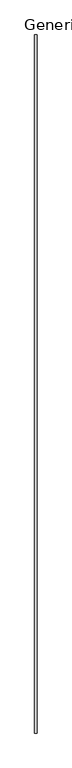
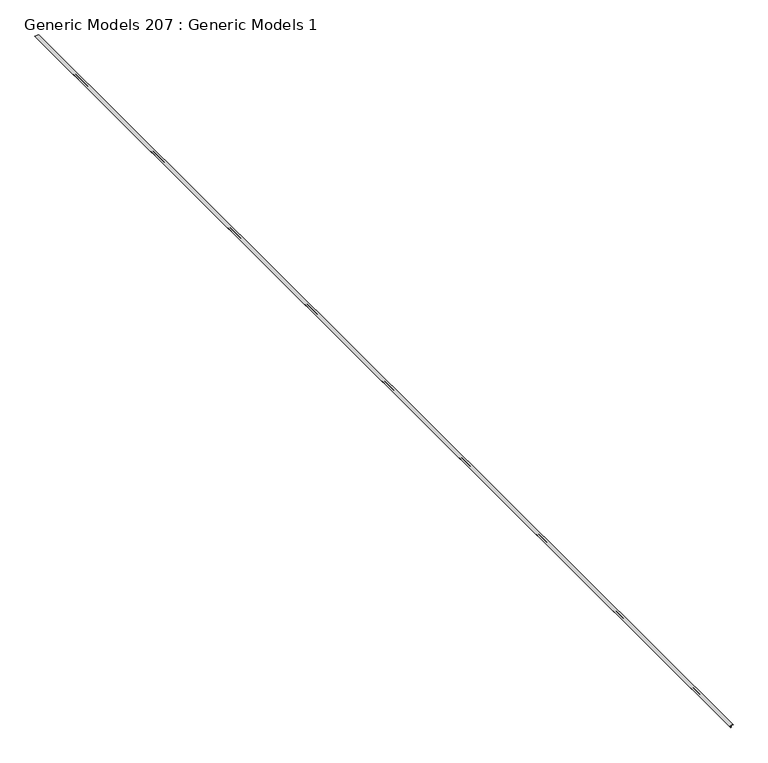
"""IFC4 building model written with IfcOpenShell, lengths in millimetres: proxy geometry, Generic Models 207 : Generic Models 1."""

from ifc_helpers import new_model, si_unit, origin, place, context, project, spatial, faceted_brep, source, transform, mapped, element, save


def generic_models_207_generic_models_1_7c4d0df2(model_context):
    return source(origin(), model_context, "Body", "Brep", [
        faceted_brep([(-8156.7486296, 11981.8769662, 126364.746), (-8156.7486296, 11981.8769662, 126363.476), (-8175.7986296, 11981.8769662, 126363.476), (-8175.7986296, 11981.8769662, 126342.521), (-8180.5484296, 11981.8769662, 126342.521), (-8180.5484296, 11981.8769662, 126343.791), (-8177.0686296, 11981.8769662, 126343.791), (-8177.0686296, 11981.8769662, 126363.476), (-8196.1186296, 11981.8769662, 126363.476), (-8196.1186296, 11981.8769662, 126364.746), (-8156.7486296, -464.1230338, 126364.746), (-8196.1186296, -464.1230338, 126364.746), (-8196.1186296, -464.1230338, 126363.476), (-8177.0686296, -464.1230338, 126363.476), (-8177.0686296, -464.1230338, 126343.791), (-8180.5484296, -464.1230338, 126343.791), (-8180.5484296, -464.1230338, 126342.521), (-8175.7986296, -464.1230338, 126342.521), (-8175.7986296, -464.1230338, 126363.476), (-8156.7486296, -464.1230338, 126363.476), (-8156.7486296, 11778.6769662, 126364.746)], [[[0, 1, 2, 3, 4, 5, 6, 7, 8, 9]], [[10, 11, 12, 13, 14, 15, 16, 17, 18, 19]], [[1, 0, 20, 10, 19]], [[2, 1, 19, 18]], [[3, 2, 18, 17]], [[4, 3, 17, 16]], [[5, 4, 16, 15]], [[6, 5, 15, 14]], [[7, 6, 14, 13]], [[8, 7, 13, 12]], [[9, 8, 12, 11]], [[0, 9, 11, 10, 20]]]),
    ])


if __name__ == "__main__":
    model = new_model("IFC4")
    model_context = context("Model", 3, world=origin())
    ifc_project = project(units=[si_unit("LENGTHUNIT", "METRE", prefix="MILLI")], contexts=[model_context])
    site = spatial("IfcSite", under=ifc_project)
    building = spatial("IfcBuilding", under=site)
    placement = place(None, origin())
    generic_models_207_generic_models_1_shape = generic_models_207_generic_models_1_7c4d0df2(model_context)
    element("IfcBuildingElementProxy", 1, Name="Generic Models 207 : Generic Models 1", ObjectType="Generic Models 207 : Generic Models 1", at=placement, inside=building, context=model_context, shape_type="MappedRepresentation", body=[
        mapped(generic_models_207_generic_models_1_shape, transform((0.0, 0.0, 0.0), x_axis=(1.0, 0.0, 0.0), y_axis=(0.0, 1.0, 0.0), z_axis=(0.0, 0.0, 1.0))),
    ])
    save(model, "model.ifc")

# Revit data of these elements
# Element 1 (IfcBuildingElementProxy, "Generic Models 207 : Generic Models 1")
#   Materials on its faces: "_16 GA. COPPER VENTED REVEAL MOLDING"
# Materials
#   "_16 GA. COPPER VENTED REVEAL MOLDING": class "Generic", colour RGB 253 192 103, transparency 0, Cost = 0
